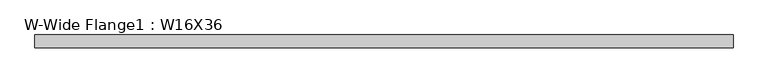
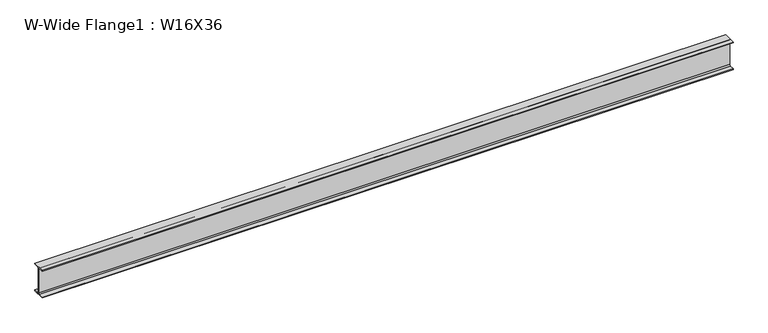
"""IFC4 building model written with IfcOpenShell, lengths in millimetres: beam geometry, W-Wide Flange1 : W16X36."""

from ifc_helpers import new_model, si_unit, point, frame, frame_2d, origin, place, context, project, spatial, polyline, circle_curve, trimmed, segment, composite_curve, outline, extrude, source, transform, mapped, element, save


def w_wide_flange1_w16x36_4a4a7409(model_context):
    return source(origin(), model_context, "Body", "SweptSolid", [
        extrude(outline(composite_curve([segment(polyline([(88.773, -191.008), (88.773, -201.93), (-88.773, -201.93), (-88.773, -191.008), (-21.3995, -191.008)]), True, "CONTINUOUS"), segment(trimmed(circle_curve(frame_2d((-21.3995, -173.355)), 17.653), [point((-21.3995, -191.008))], [point((-3.7465, -173.355))], True, "CARTESIAN"), True, "CONTINUOUS"), segment(polyline([(-3.7465, -173.355), (-3.7465, 173.355)]), True, "CONTINUOUS"), segment(trimmed(circle_curve(frame_2d((-21.3995, 173.355)), 17.653), [point((-3.7465, 173.355))], [point((-21.3995, 191.008))], True, "CARTESIAN"), True, "CONTINUOUS"), segment(polyline([(-21.3995, 191.008), (-88.773, 191.008), (-88.773, 201.93), (88.773, 201.93), (88.773, 191.008), (21.3995, 191.008)]), True, "CONTINUOUS"), segment(trimmed(circle_curve(frame_2d((21.3995, 173.355)), 17.653), [point((21.3995, 191.008))], [point((3.7465, 173.355))], True, "CARTESIAN"), True, "CONTINUOUS"), segment(polyline([(3.7465, 173.355), (3.7465, -173.355)]), True, "CONTINUOUS"), segment(trimmed(circle_curve(frame_2d((21.3995, -173.355)), 17.653), [point((3.7465, -173.355))], [point((21.3995, -191.008))], True, "CARTESIAN"), True, "CONTINUOUS"), segment(polyline([(21.3995, -191.008), (88.773, -191.008)]), True, "CONTINUOUS")], self_intersect=False)), frame((-4803.15, 0.0, 0.0), z_axis=(1.0, 0.0, 0.0), x_axis=(0.0, 1.0, 0.0)), (0.0, 0.0, 1.0), 9606.3),
    ])


if __name__ == "__main__":
    model = new_model("IFC4")
    model_context = context("Model", 3, world=origin())
    ifc_project = project(units=[si_unit("LENGTHUNIT", "METRE", prefix="MILLI")], contexts=[model_context])
    site = spatial("IfcSite", under=ifc_project)
    building = spatial("IfcBuilding", under=site)
    placement = place(None, origin())
    w_wide_flange1_w16x36_shape = w_wide_flange1_w16x36_4a4a7409(model_context)
    element("IfcBeam", 1, ObjectType="W-Wide Flange1 : W16X36", at=placement, inside=building, context=model_context, shape_type="MappedRepresentation", body=[
        mapped(w_wide_flange1_w16x36_shape, transform((0.0, 0.0, 0.0), x_axis=(1.0, 0.0, 0.0), y_axis=(0.0, 1.0, 0.0), z_axis=(0.0, 0.0, 1.0))),
    ])
    save(model, "model.ifc")

# Revit data of these elements
# Type "W-Wide Flange1 : W16X36"
#   Assembly Code = "B10"
#   W = 36
#   Start Extension Calculation [instance default] = 10' - 0"
#   Start Extension [instance default] = -0' - 0 1/2"
#   End Extension Calculation [instance default] = 10' - 0"
#   End Extension [instance default] = -0' - 0 1/2"
#   Length [instance default] = 5' - 0"
#   bf = 0' - 6.99"
#   d = 1' - 3.9"
#   k = 0' - 1 1/8"
#   k2 = 0' - 0.695"
#   tf = 0' - 0.43"
#   tw = 0' - 0.295"
#   A = 0.0736111 SF
#   Structural Material [instance default] = Metal - Steel - ASTM A992
# Element 1 (IfcBeam, "W-Wide Flange1 : W16X36")
#   Materials on its faces: "Metal - Steel - ASTM A992"
# Materials
#   "Metal - Steel - ASTM A992": class "Metal", colour RGB 199 199 199, transparency 0
